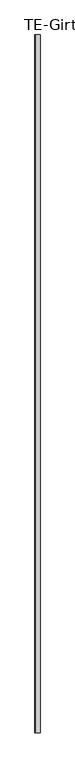
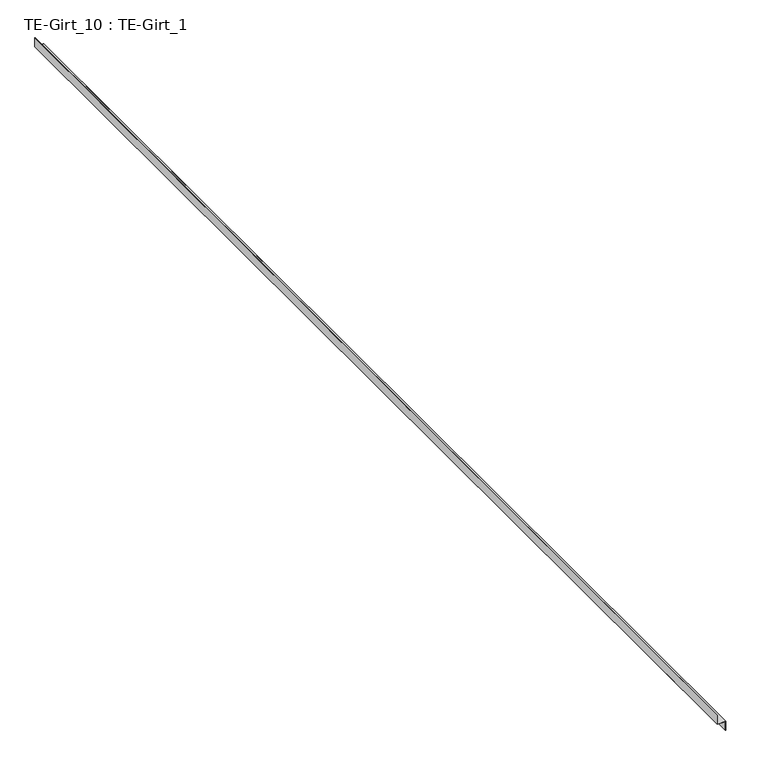
"""IFC4 building model written with IfcOpenShell, lengths in millimetres: proxy geometry, TE-Girt_10 : TE-Girt_1."""

import ifcopenshell
import ifcopenshell.guid

model = None  # the IFC model being written
_history = None  # IfcOwnerHistory: only IFC2X3 demands one
_inside = {}  # id of a spatial element -> (the spatial element, [elements in it])
_under = {}  # id of a project, library or spatial element -> (it, [spatial elements below it])
_declared = {}  # id of a project -> (the project, [libraries it declares])
_typed = {}  # id of a type object -> (the type object, [elements of that type])
_made_of = {}  # id of a material, layer set ... -> (it, [elements and type objects made of it])


def new_model(schema):
    """Start an empty IFC model of exactly this schema.

    Asked for "IFC4X3", IfcOpenShell would pick the latest addendum, in which some entities
    have other attributes; the version numbers below select the first issue.
    IFC2X3 requires an IfcOwnerHistory on every rooted entity: one is made here for all.
    """
    global model, _history
    if schema == "IFC4X3":
        model = ifcopenshell.file(schema_version=(4, 3, 0, 0))
    else:
        model = ifcopenshell.file(schema=schema)
    _inside.clear()
    _under.clear()
    _declared.clear()
    _typed.clear()
    _made_of.clear()
    _history = None
    if model.schema == "IFC2X3":
        org = make("IfcOrganization", Name="unknown")
        user = make(
            "IfcPersonAndOrganization",
            ThePerson=make("IfcPerson", FamilyName="unknown"),
            TheOrganization=org,
        )
        app = make(
            "IfcApplication",
            ApplicationDeveloper=org,
            Version="unknown",
            ApplicationFullName="unknown",
            ApplicationIdentifier="unknown",
        )
        _history = make(
            "IfcOwnerHistory",
            OwningUser=user,
            OwningApplication=app,
            ChangeAction="ADDED",
            CreationDate=0,
        )
    return model


def make(cls, **values):
    """One entity of the class cls with the attributes given. An attribute that is None is left unset."""
    return model.create_entity(
        cls, **{name: value for name, value in values.items() if value is not None}
    )


def rooted(cls, **values):
    """An entity with a GlobalId (a new one), such as an element, a storey or a relation."""
    return make(cls, GlobalId=ifcopenshell.guid.new(), OwnerHistory=_history, **values)


def si_unit(unit_type, name, prefix=None):
    """IfcSIUnit, for example si_unit("LENGTHUNIT", "METRE", prefix="MILLI")."""
    return make("IfcSIUnit", UnitType=unit_type, Prefix=prefix, Name=name)


def assignment(units):
    """IfcUnitAssignment: the units of a project."""
    return None if units is None else make("IfcUnitAssignment", Units=units)


def point(xyz):
    """IfcCartesianPoint."""
    return None if xyz is None else make("IfcCartesianPoint", Coordinates=xyz)


def direction(xyz):
    """IfcDirection."""
    return None if xyz is None else make("IfcDirection", DirectionRatios=xyz)


def frame(location, z_axis=None, x_axis=None):
    """IfcAxis2Placement3D, a coordinate frame: its origin and axes. An axis left out is left unset."""
    return make(
        "IfcAxis2Placement3D",
        Location=point(location),
        Axis=direction(z_axis),
        RefDirection=direction(x_axis),
    )


def origin():
    """The frame at (0, 0, 0) with its axes left unset."""
    return frame((0.0, 0.0, 0.0))


def place(relative_to, where):
    """IfcLocalPlacement: puts the frame where relative to a parent placement (None: the world)."""
    return make(
        "IfcLocalPlacement", PlacementRelTo=relative_to, RelativePlacement=where
    )


def context(
    kind, dimensions, precision=None, world=None, true_north=None, identifier=None
):
    """IfcGeometricRepresentationContext, for example the 3D "Model" context."""
    return make(
        "IfcGeometricRepresentationContext",
        ContextIdentifier=identifier,
        ContextType=kind,
        CoordinateSpaceDimension=dimensions,
        Precision=precision,
        WorldCoordinateSystem=world,
        TrueNorth=true_north,
    )


def project(units=None, contexts=None):
    """IfcProject with its units and contexts."""
    return rooted(
        "IfcProject",
        Name="project",
        RepresentationContexts=contexts,
        UnitsInContext=assignment(units),
    )


def spatial(cls, under=None, at=None, **own):
    """A site, building, storey or space (cls), placed at a placement, below another one or the project."""
    s = rooted(cls, ObjectPlacement=at, **own)
    if under is not None:
        _under.setdefault(under.id(), (under, []))[1].append(s)
    return s


def polyline(points):
    """IfcPolyline through the points."""
    return make("IfcPolyline", Points=[point(p) for p in points])


def outline(outer, holes=None, kind="AREA"):
    """IfcArbitraryClosedProfileDef: a profile drawn as a closed curve; with holes, ...WithVoids."""
    if holes is None:
        return make("IfcArbitraryClosedProfileDef", ProfileType=kind, OuterCurve=outer)
    return make(
        "IfcArbitraryProfileDefWithVoids",
        ProfileType=kind,
        OuterCurve=outer,
        InnerCurves=holes,
    )


def extrude(swept, where, along, depth):
    """IfcExtrudedAreaSolid: the profile swept, set in the frame where, extruded along a direction by depth."""
    return make(
        "IfcExtrudedAreaSolid",
        SweptArea=swept,
        Position=where,
        ExtrudedDirection=direction(along),
        Depth=depth,
    )


def shape(context_of_items, identifier, shape_type, items):
    """IfcShapeRepresentation: the items that make up one representation, for example the "Body"."""
    return make(
        "IfcShapeRepresentation",
        ContextOfItems=context_of_items,
        RepresentationIdentifier=identifier,
        RepresentationType=shape_type,
        Items=items,
    )


def source(mapping_origin, context_of_items, identifier, shape_type, items):
    """IfcRepresentationMap: a shape defined once, which mapped items show again and again."""
    return make(
        "IfcRepresentationMap",
        MappingOrigin=mapping_origin,
        MappedRepresentation=shape(context_of_items, identifier, shape_type, items),
    )


def transform(
    local_origin,
    x_axis=None,
    y_axis=None,
    z_axis=None,
    scale=None,
    scale2=None,
    scale3=None,
    uniform=True,
):
    """IfcCartesianTransformationOperator3D, or its non-uniform kind. x_axis, y_axis, z_axis: its Axis1, 2, 3."""
    if uniform:
        return make(
            "IfcCartesianTransformationOperator3D",
            Axis1=direction(x_axis),
            Axis2=direction(y_axis),
            LocalOrigin=point(local_origin),
            Scale=scale,
            Axis3=direction(z_axis),
        )
    return make(
        "IfcCartesianTransformationOperator3DnonUniform",
        Axis1=direction(x_axis),
        Axis2=direction(y_axis),
        LocalOrigin=point(local_origin),
        Scale=scale,
        Axis3=direction(z_axis),
        Scale2=scale2,
        Scale3=scale3,
    )


def mapped(mapping_source, mapping_target):
    """IfcMappedItem: shows the shape of a source again, moved by a transform."""
    return make(
        "IfcMappedItem", MappingSource=mapping_source, MappingTarget=mapping_target
    )


def made_of(thing, what):
    """Note that an element or type object is made of a material, layer set ...; save() writes the relation."""
    if what is not None:
        _made_of.setdefault(what.id(), (what, []))[1].append(thing)
    return thing


def element(
    cls,
    number,
    at=None,
    inside=None,
    cuts=None,
    type_object=None,
    material=None,
    context=None,
    identifier="Body",
    shape_type=None,
    held_by="IfcProductDefinitionShape",
    body=None,
    shapes=None,
    **own,
):
    """One element of the class cls, such as IfcWall. Its Tag is "e" and its number.

    at: its placement. inside: the storey or other place that contains it. cuts: it is an
    opening in that element (IfcRelVoidsElement). A single representation is given by context,
    identifier, shape_type and body (its items); several are given by shapes. held_by: the class
    of the entity that holds the representations. save() writes the other relations.
    """
    e = rooted(cls, Tag="e%d" % number, ObjectPlacement=at, **own)
    if body is not None:
        shapes = [shape(context, identifier, shape_type, body)]
    if shapes is not None:
        e.Representation = make(held_by, Representations=shapes)
    if inside is not None:
        _inside.setdefault(inside.id(), (inside, []))[1].append(e)
    if cuts is not None:
        rooted(
            "IfcRelVoidsElement", RelatingBuildingElement=cuts, RelatedOpeningElement=e
        )
    if type_object is not None:
        _typed.setdefault(type_object.id(), (type_object, []))[1].append(e)
    return made_of(e, material)


def aggregate(whole, parts):
    """IfcRelAggregates: a whole, such as a stair, and the parts it consists of."""
    return rooted("IfcRelAggregates", RelatingObject=whole, RelatedObjects=parts)


def save(model, path):
    """Write the relations noted so far, then the file.

    IfcRelAggregates (storeys below a building ...), IfcRelContainedInSpatialStructure (elements
    in a storey), IfcRelDefinesByType, IfcRelAssociatesMaterial and IfcRelDeclares: one each for
    every whole, place, type object, material and project.
    """
    for whole, parts in _under.values():
        aggregate(whole, parts)
    for where, things in _inside.values():
        rooted(
            "IfcRelContainedInSpatialStructure",
            RelatedElements=things,
            RelatingStructure=where,
        )
    for kind, things in _typed.values():
        rooted("IfcRelDefinesByType", RelatedObjects=things, RelatingType=kind)
    for what, things in _made_of.values():
        rooted("IfcRelAssociatesMaterial", RelatedObjects=things, RelatingMaterial=what)
    for by, libraries in _declared.values():
        rooted("IfcRelDeclares", RelatingContext=by, RelatedDefinitions=libraries)
    model.write(path)


def te_girt_10_te_girt_1_95d38daf(model_context):
    return source(origin(), model_context, "Body", "SweptSolid", [
        extrude(outline(polyline([(844.55, 590353.5520246), (844.55, 590319.5364427), (881.7570313, 590319.5364427), (881.7570313, 590318.6434739), (843.6570313, 590318.6434739), (843.6570313, 590352.6590559), (806.45, 590352.6590559), (806.45, 590353.5520246), (844.55, 590353.5520246)])), frame((0.0, -536417.5913841, 0.0), z_axis=(0.0, 1.0, 0.0), x_axis=(0.0, 0.0, 1.0)), (0.0, 0.0, 1.0), 4778.375),
    ])


if __name__ == "__main__":
    model = new_model("IFC4")
    model_context = context("Model", 3, world=origin())
    ifc_project = project(units=[si_unit("LENGTHUNIT", "METRE", prefix="MILLI")], contexts=[model_context])
    site = spatial("IfcSite", under=ifc_project)
    building = spatial("IfcBuilding", under=site)
    placement = place(None, origin())
    te_girt_10_te_girt_1_shape = te_girt_10_te_girt_1_95d38daf(model_context)
    element("IfcBuildingElementProxy", 1, Name="TE-Girt_10 : TE-Girt_1", ObjectType="TE-Girt_10 : TE-Girt_1", at=placement, inside=building, context=model_context, shape_type="MappedRepresentation", body=[
        mapped(te_girt_10_te_girt_1_shape, transform((0.0, 0.0, 0.0), x_axis=(1.0, 0.0, 0.0), y_axis=(0.0, 1.0, 0.0), z_axis=(0.0, 0.0, 1.0))),
    ])
    save(model, "model.ifc")

# Revit data of these elements
# Element 1 (IfcBuildingElementProxy, "TE-Girt_10 : TE-Girt_1")
#   Materials on its faces: "Z-FURRING, COLD-FORMED GALV."
# Materials
#   "Z-FURRING, COLD-FORMED GALV.": class "Generic", colour RGB 143 142 141, transparency 0, Cost = 0
